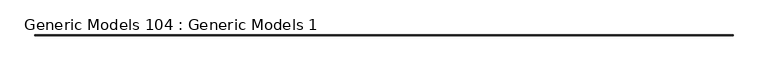
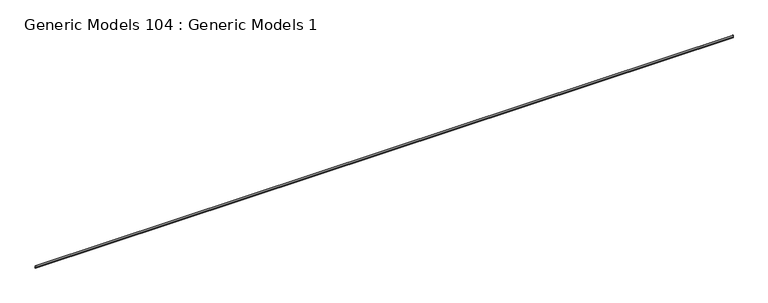
"""IFC4 building model written with IfcOpenShell, lengths in millimetres: proxy geometry, Generic Models 104 : Generic Models 1."""

from ifc_helpers import new_model, si_unit, frame, origin, place, context, project, spatial, polyline, outline, extrude, source, transform, mapped, element, save


def generic_models_104_generic_models_1_58ad6d10(model_context):
    return source(origin(), model_context, "Body", "SweptSolid", [
        extrude(outline(polyline([(51501.1226718, 126996.7728942), (51480.9690553, 126990.2949461), (51480.1457344, 126985.9229543), (51478.8976718, 126986.1579859), (51479.8608669, 126991.2727363), (51496.9724696, 126996.7728942), (51478.8976718, 127002.5826506), (51478.8976718, 127047.5728942), (51480.1676718, 127047.5728942), (51480.1676718, 127003.50843), (51501.1226718, 126996.7728942)])), frame((-20998.9733045, 0.0, 0.0), z_axis=(1.0, 0.0, 0.0), x_axis=(0.0, 1.0, 0.0)), (0.0, 0.0, 1.0), 19050.0),
    ])


if __name__ == "__main__":
    model = new_model("IFC4")
    model_context = context("Model", 3, world=origin())
    ifc_project = project(units=[si_unit("LENGTHUNIT", "METRE", prefix="MILLI")], contexts=[model_context])
    site = spatial("IfcSite", under=ifc_project)
    building = spatial("IfcBuilding", under=site)
    placement = place(None, origin())
    generic_models_104_generic_models_1_shape = generic_models_104_generic_models_1_58ad6d10(model_context)
    element("IfcBuildingElementProxy", 1, Name="Generic Models 104 : Generic Models 1", ObjectType="Generic Models 104 : Generic Models 1", at=placement, inside=building, context=model_context, shape_type="MappedRepresentation", body=[
        mapped(generic_models_104_generic_models_1_shape, transform((0.0, 0.0, 0.0), x_axis=(1.0, 0.0, 0.0), y_axis=(0.0, 1.0, 0.0), z_axis=(0.0, 0.0, 1.0))),
    ])
    save(model, "model.ifc")

# Revit data of these elements
# Element 1 (IfcBuildingElementProxy, "Generic Models 104 : Generic Models 1")
#   Materials on its faces: "_16 GA. COPPER WEEP SCREED W/ MIN. 3 1/2\" ATTACHEMENT FLANGE - LAP UNDERLAYMENT OVER WEED SCREED"
# Materials
#   "_16 GA. COPPER WEEP SCREED W/ MIN. 3 1/2\" ATTACHEMENT FLANGE - LAP UNDERLAYMENT OVER WEED SCREED": class "Generic", colour RGB 253 192 103, transparency 0, Cost = 0
